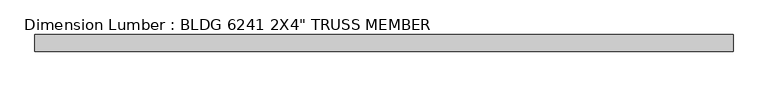
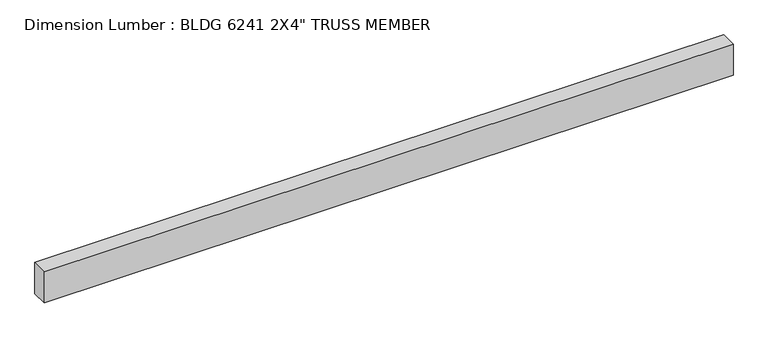
"""IFC4 building model written with IfcOpenShell, lengths in millimetres: beam geometry."""

from ifc_helpers import new_model, si_unit, frame, origin, place, context, project, spatial, polyline, outline, extrude, source, transform, mapped, element, save


def beam_4f4e5714(model_context):
    return source(origin(), model_context, "Body", "SweptSolid", [
        extrude(outline(polyline([(1066.8, 25.4), (1066.8, -25.4), (-1066.8, -25.4), (-1066.8, 25.4), (1066.8, 25.4)])), frame((0.0, 0.0, -50.8), z_axis=(0.0, 0.0, 1.0), x_axis=(1.0, 0.0, 0.0)), (0.0, 0.0, 1.0), 101.6),
    ])


if __name__ == "__main__":
    model = new_model("IFC4")
    model_context = context("Model", 3, world=origin())
    ifc_project = project(units=[si_unit("LENGTHUNIT", "METRE", prefix="MILLI")], contexts=[model_context])
    site = spatial("IfcSite", under=ifc_project)
    building = spatial("IfcBuilding", under=site)
    placement = place(None, origin())
    beam_shape = beam_4f4e5714(model_context)
    element("IfcBeam", 1, ObjectType="Dimension Lumber : BLDG 6241 2X4\" TRUSS MEMBER", at=placement, inside=building, context=model_context, shape_type="MappedRepresentation", body=[
        mapped(beam_shape, transform((0.0, 0.0, 0.0), x_axis=(1.0, 0.0, 0.0), y_axis=(0.0, 1.0, 0.0), z_axis=(0.0, 0.0, 1.0))),
    ])
    save(model, "model.ifc")

# Revit data of these elements
# Type "Dimension Lumber : BLDG 6241 2X4\" TRUSS MEMBER"
#   Assembly Code = "B10"
#   A = 0.273472 SF
#   Length [instance default] = 5' - 0"
#   b = 0' - 2"
#   d = 0' - 4"
#   Structural Material [instance default] = Softwood, Lumber
# Element 1 (IfcBeam, "Dimension Lumber : BLDG 6241 2X4\" TRUSS MEMBER")
#   Materials on its faces: "Softwood, Lumber"
# Materials
#   "Softwood, Lumber": class "Wood", colour RGB 223 192 134, transparency 0, Description = "Pinus Echinata", Cost = 0
